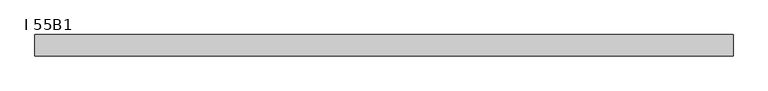
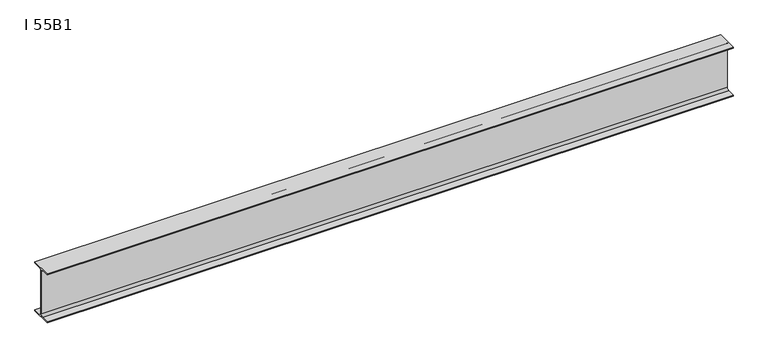
"""IFC4 building model written with IfcOpenShell, lengths in millimetres: beam geometry, Типовая двутавровая балка (АСТО 20-93) Балки : I 55B1."""

from ifc_helpers import new_model, si_unit, point, frame, frame_2d, origin, place, context, project, spatial, polyline, circle_curve, trimmed, segment, composite_curve, outline, extrude, source, transform, mapped, element, save


def i_55b1_cd40b888(model_context):
    return source(origin(), model_context, "Body", "SweptSolid", [
        extrude(outline(composite_curve([segment(polyline([(110.0, -258.0), (110.0, -271.5), (-110.0, -271.5), (-110.0, -258.0), (-28.75, -258.0)]), True, "CONTINUOUS"), segment(trimmed(circle_curve(frame_2d((-28.75, -234.0)), 24.0), [point((-28.75, -258.0))], [point((-4.75, -234.0))], True, "CARTESIAN"), True, "CONTINUOUS"), segment(polyline([(-4.75, -234.0), (-4.75, 234.0)]), True, "CONTINUOUS"), segment(trimmed(circle_curve(frame_2d((-28.75, 234.0)), 24.0), [point((-4.75, 234.0))], [point((-28.75, 258.0))], True, "CARTESIAN"), True, "CONTINUOUS"), segment(polyline([(-28.75, 258.0), (-110.0, 258.0), (-110.0, 271.5), (110.0, 271.5), (110.0, 258.0), (28.75, 258.0)]), True, "CONTINUOUS"), segment(trimmed(circle_curve(frame_2d((28.75, 234.0)), 24.0), [point((28.75, 258.0))], [point((4.75, 234.0))], True, "CARTESIAN"), True, "CONTINUOUS"), segment(polyline([(4.75, 234.0), (4.75, -234.0)]), True, "CONTINUOUS"), segment(trimmed(circle_curve(frame_2d((28.75, -234.0)), 24.0), [point((4.75, -234.0))], [point((28.75, -258.0))], True, "CARTESIAN"), True, "CONTINUOUS"), segment(polyline([(28.75, -258.0), (110.0, -258.0)]), True, "CONTINUOUS")], self_intersect=False)), frame((-3576.0, 0.0, 0.0), z_axis=(1.0, 0.0, 0.0), x_axis=(0.0, 1.0, 0.0)), (0.0, 0.0, 1.0), 7152.0),
    ])


if __name__ == "__main__":
    model = new_model("IFC4")
    model_context = context("Model", 3, world=origin())
    ifc_project = project(units=[si_unit("LENGTHUNIT", "METRE", prefix="MILLI")], contexts=[model_context])
    site = spatial("IfcSite", under=ifc_project)
    building = spatial("IfcBuilding", under=site)
    placement = place(None, origin())
    i_55b1_shape = i_55b1_cd40b888(model_context)
    element("IfcBeam", 1, ObjectType="Типовая двутавровая балка (АСТО 20-93) Балки : I 55B1", at=placement, inside=building, context=model_context, shape_type="MappedRepresentation", body=[
        mapped(i_55b1_shape, transform((0.0, 0.0, 0.0), x_axis=(1.0, 0.0, 0.0), y_axis=(0.0, 1.0, 0.0), z_axis=(0.0, 0.0, 1.0))),
    ])
    save(model, "model.ifc")

# Revit data of these elements
# Type "Типовая двутавровая балка (АСТО 20-93) Балки : I 55B1"
#   ra = 24 mm
#   W = 0.872792
#   Vz = 271.5 mm
#   Vy = 110 mm
#   Vpz = 271.5 mm
#   Vpy = 110 mm
#   Length [instance default] = 1500 mm
#   bf = 220 mm
#   d = 543 mm
#   tf = 13.5 mm
#   tw = 9.5 mm
#   A = 0.011336 m²
#   Structural Material [instance default] = Металл - Сталь - 345 МПa
#   Assembly Code = ""
# Element 1 (IfcBeam, "Типовая двутавровая балка (АСТО 20-93) Балки : I 55B1")
#   Structural Material = C235
#   Materials on its faces: "C235"
# Materials
#   "Металл - Сталь - 345 МПa": class "Металл", colour RGB 247 247 247, transparency 0
#   "C235": class "Не назначено", colour RGB 0 0 0, transparency 0
